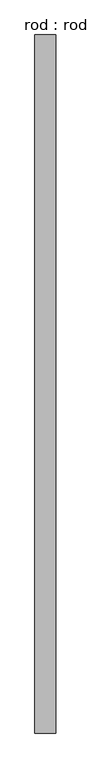
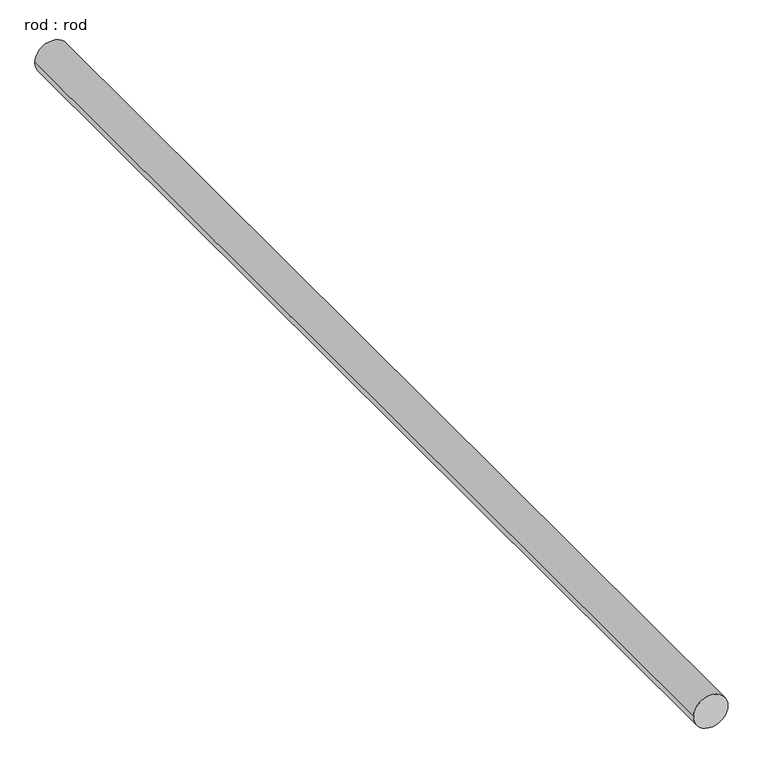
"""IFC4 building model written with IfcOpenShell, lengths in millimetres: proxy geometry, rod : rod."""

import ifcopenshell
import ifcopenshell.guid

model = None  # the IFC model being written
_history = None  # IfcOwnerHistory: only IFC2X3 demands one
_inside = {}  # id of a spatial element -> (the spatial element, [elements in it])
_under = {}  # id of a project, library or spatial element -> (it, [spatial elements below it])
_declared = {}  # id of a project -> (the project, [libraries it declares])
_typed = {}  # id of a type object -> (the type object, [elements of that type])
_made_of = {}  # id of a material, layer set ... -> (it, [elements and type objects made of it])


def new_model(schema):
    """Start an empty IFC model of exactly this schema.

    Asked for "IFC4X3", IfcOpenShell would pick the latest addendum, in which some entities
    have other attributes; the version numbers below select the first issue.
    IFC2X3 requires an IfcOwnerHistory on every rooted entity: one is made here for all.
    """
    global model, _history
    if schema == "IFC4X3":
        model = ifcopenshell.file(schema_version=(4, 3, 0, 0))
    else:
        model = ifcopenshell.file(schema=schema)
    _inside.clear()
    _under.clear()
    _declared.clear()
    _typed.clear()
    _made_of.clear()
    _history = None
    if model.schema == "IFC2X3":
        org = make("IfcOrganization", Name="unknown")
        user = make(
            "IfcPersonAndOrganization",
            ThePerson=make("IfcPerson", FamilyName="unknown"),
            TheOrganization=org,
        )
        app = make(
            "IfcApplication",
            ApplicationDeveloper=org,
            Version="unknown",
            ApplicationFullName="unknown",
            ApplicationIdentifier="unknown",
        )
        _history = make(
            "IfcOwnerHistory",
            OwningUser=user,
            OwningApplication=app,
            ChangeAction="ADDED",
            CreationDate=0,
        )
    return model


def make(cls, **values):
    """One entity of the class cls with the attributes given. An attribute that is None is left unset."""
    return model.create_entity(
        cls, **{name: value for name, value in values.items() if value is not None}
    )


def rooted(cls, **values):
    """An entity with a GlobalId (a new one), such as an element, a storey or a relation."""
    return make(cls, GlobalId=ifcopenshell.guid.new(), OwnerHistory=_history, **values)


def si_unit(unit_type, name, prefix=None):
    """IfcSIUnit, for example si_unit("LENGTHUNIT", "METRE", prefix="MILLI")."""
    return make("IfcSIUnit", UnitType=unit_type, Prefix=prefix, Name=name)


def assignment(units):
    """IfcUnitAssignment: the units of a project."""
    return None if units is None else make("IfcUnitAssignment", Units=units)


def point(xyz):
    """IfcCartesianPoint."""
    return None if xyz is None else make("IfcCartesianPoint", Coordinates=xyz)


def direction(xyz):
    """IfcDirection."""
    return None if xyz is None else make("IfcDirection", DirectionRatios=xyz)


def frame(location, z_axis=None, x_axis=None):
    """IfcAxis2Placement3D, a coordinate frame: its origin and axes. An axis left out is left unset."""
    return make(
        "IfcAxis2Placement3D",
        Location=point(location),
        Axis=direction(z_axis),
        RefDirection=direction(x_axis),
    )


def frame_2d(location, x_axis=None):
    """IfcAxis2Placement2D, a coordinate frame in the plane: its origin and x axis."""
    return make(
        "IfcAxis2Placement2D", Location=point(location), RefDirection=direction(x_axis)
    )


def origin():
    """The frame at (0, 0, 0) with its axes left unset."""
    return frame((0.0, 0.0, 0.0))


def place(relative_to, where):
    """IfcLocalPlacement: puts the frame where relative to a parent placement (None: the world)."""
    return make(
        "IfcLocalPlacement", PlacementRelTo=relative_to, RelativePlacement=where
    )


def context(
    kind, dimensions, precision=None, world=None, true_north=None, identifier=None
):
    """IfcGeometricRepresentationContext, for example the 3D "Model" context."""
    return make(
        "IfcGeometricRepresentationContext",
        ContextIdentifier=identifier,
        ContextType=kind,
        CoordinateSpaceDimension=dimensions,
        Precision=precision,
        WorldCoordinateSystem=world,
        TrueNorth=true_north,
    )


def project(units=None, contexts=None):
    """IfcProject with its units and contexts."""
    return rooted(
        "IfcProject",
        Name="project",
        RepresentationContexts=contexts,
        UnitsInContext=assignment(units),
    )


def spatial(cls, under=None, at=None, **own):
    """A site, building, storey or space (cls), placed at a placement, below another one or the project."""
    s = rooted(cls, ObjectPlacement=at, **own)
    if under is not None:
        _under.setdefault(under.id(), (under, []))[1].append(s)
    return s


def circle_curve(where, radius):
    """IfcCircle in the frame where."""
    return make("IfcCircle", Position=where, Radius=radius)


def trimmed(basis, trim1, trim2, sense, master):
    """IfcTrimmedCurve: the piece of a basis curve between two trims."""
    return make(
        "IfcTrimmedCurve",
        BasisCurve=basis,
        Trim1=trim1,
        Trim2=trim2,
        SenseAgreement=sense,
        MasterRepresentation=master,
    )


def segment(curve, same_sense, transition):
    """IfcCompositeCurveSegment."""
    return make(
        "IfcCompositeCurveSegment",
        Transition=transition,
        SameSense=same_sense,
        ParentCurve=curve,
    )


def composite_curve(segments, self_intersect=None):
    """IfcCompositeCurve: segments joined end to end."""
    return make("IfcCompositeCurve", Segments=segments, SelfIntersect=self_intersect)


def outline(outer, holes=None, kind="AREA"):
    """IfcArbitraryClosedProfileDef: a profile drawn as a closed curve; with holes, ...WithVoids."""
    if holes is None:
        return make("IfcArbitraryClosedProfileDef", ProfileType=kind, OuterCurve=outer)
    return make(
        "IfcArbitraryProfileDefWithVoids",
        ProfileType=kind,
        OuterCurve=outer,
        InnerCurves=holes,
    )


def extrude(swept, where, along, depth):
    """IfcExtrudedAreaSolid: the profile swept, set in the frame where, extruded along a direction by depth."""
    return make(
        "IfcExtrudedAreaSolid",
        SweptArea=swept,
        Position=where,
        ExtrudedDirection=direction(along),
        Depth=depth,
    )


def shape(context_of_items, identifier, shape_type, items):
    """IfcShapeRepresentation: the items that make up one representation, for example the "Body"."""
    return make(
        "IfcShapeRepresentation",
        ContextOfItems=context_of_items,
        RepresentationIdentifier=identifier,
        RepresentationType=shape_type,
        Items=items,
    )


def source(mapping_origin, context_of_items, identifier, shape_type, items):
    """IfcRepresentationMap: a shape defined once, which mapped items show again and again."""
    return make(
        "IfcRepresentationMap",
        MappingOrigin=mapping_origin,
        MappedRepresentation=shape(context_of_items, identifier, shape_type, items),
    )


def transform(
    local_origin,
    x_axis=None,
    y_axis=None,
    z_axis=None,
    scale=None,
    scale2=None,
    scale3=None,
    uniform=True,
):
    """IfcCartesianTransformationOperator3D, or its non-uniform kind. x_axis, y_axis, z_axis: its Axis1, 2, 3."""
    if uniform:
        return make(
            "IfcCartesianTransformationOperator3D",
            Axis1=direction(x_axis),
            Axis2=direction(y_axis),
            LocalOrigin=point(local_origin),
            Scale=scale,
            Axis3=direction(z_axis),
        )
    return make(
        "IfcCartesianTransformationOperator3DnonUniform",
        Axis1=direction(x_axis),
        Axis2=direction(y_axis),
        LocalOrigin=point(local_origin),
        Scale=scale,
        Axis3=direction(z_axis),
        Scale2=scale2,
        Scale3=scale3,
    )


def mapped(mapping_source, mapping_target):
    """IfcMappedItem: shows the shape of a source again, moved by a transform."""
    return make(
        "IfcMappedItem", MappingSource=mapping_source, MappingTarget=mapping_target
    )


def made_of(thing, what):
    """Note that an element or type object is made of a material, layer set ...; save() writes the relation."""
    if what is not None:
        _made_of.setdefault(what.id(), (what, []))[1].append(thing)
    return thing


def element(
    cls,
    number,
    at=None,
    inside=None,
    cuts=None,
    type_object=None,
    material=None,
    context=None,
    identifier="Body",
    shape_type=None,
    held_by="IfcProductDefinitionShape",
    body=None,
    shapes=None,
    **own,
):
    """One element of the class cls, such as IfcWall. Its Tag is "e" and its number.

    at: its placement. inside: the storey or other place that contains it. cuts: it is an
    opening in that element (IfcRelVoidsElement). A single representation is given by context,
    identifier, shape_type and body (its items); several are given by shapes. held_by: the class
    of the entity that holds the representations. save() writes the other relations.
    """
    e = rooted(cls, Tag="e%d" % number, ObjectPlacement=at, **own)
    if body is not None:
        shapes = [shape(context, identifier, shape_type, body)]
    if shapes is not None:
        e.Representation = make(held_by, Representations=shapes)
    if inside is not None:
        _inside.setdefault(inside.id(), (inside, []))[1].append(e)
    if cuts is not None:
        rooted(
            "IfcRelVoidsElement", RelatingBuildingElement=cuts, RelatedOpeningElement=e
        )
    if type_object is not None:
        _typed.setdefault(type_object.id(), (type_object, []))[1].append(e)
    return made_of(e, material)


def aggregate(whole, parts):
    """IfcRelAggregates: a whole, such as a stair, and the parts it consists of."""
    return rooted("IfcRelAggregates", RelatingObject=whole, RelatedObjects=parts)


def save(model, path):
    """Write the relations noted so far, then the file.

    IfcRelAggregates (storeys below a building ...), IfcRelContainedInSpatialStructure (elements
    in a storey), IfcRelDefinesByType, IfcRelAssociatesMaterial and IfcRelDeclares: one each for
    every whole, place, type object, material and project.
    """
    for whole, parts in _under.values():
        aggregate(whole, parts)
    for where, things in _inside.values():
        rooted(
            "IfcRelContainedInSpatialStructure",
            RelatedElements=things,
            RelatingStructure=where,
        )
    for kind, things in _typed.values():
        rooted("IfcRelDefinesByType", RelatedObjects=things, RelatingType=kind)
    for what, things in _made_of.values():
        rooted("IfcRelAssociatesMaterial", RelatedObjects=things, RelatingMaterial=what)
    for by, libraries in _declared.values():
        rooted("IfcRelDeclares", RelatingContext=by, RelatedDefinitions=libraries)
    model.write(path)


def rod_rod_481c27a9(model_context):
    return source(origin(), model_context, "Body", "SweptSolid", [
        extrude(outline(composite_curve([segment(trimmed(circle_curve(frame_2d((0.0108462, 0.0)), 200.0), [point((0.0108462, 200.0))], [point((0.0108462, -200.0))], False, "CARTESIAN"), True, "CONTINUOUS"), segment(trimmed(circle_curve(frame_2d((0.0108462, 0.0)), 200.0), [point((0.0108462, -200.0))], [point((0.0108462, 200.0))], False, "CARTESIAN"), True, "CONTINUOUS")], self_intersect=False)), frame((0.0, -2557.2713847, 0.0), z_axis=(0.0, 1.0, 0.0), x_axis=(0.0, 0.0, 1.0)), (0.0, 0.0, 1.0), 13300.0),
    ])


if __name__ == "__main__":
    model = new_model("IFC4")
    model_context = context("Model", 3, world=origin())
    ifc_project = project(units=[si_unit("LENGTHUNIT", "METRE", prefix="MILLI")], contexts=[model_context])
    site = spatial("IfcSite", under=ifc_project)
    building = spatial("IfcBuilding", under=site)
    placement = place(None, origin())
    rod_rod_shape = rod_rod_481c27a9(model_context)
    element("IfcBuildingElementProxy", 1, Name="rod : rod", ObjectType="rod : rod", at=placement, inside=building, context=model_context, shape_type="MappedRepresentation", body=[
        mapped(rod_rod_shape, transform((0.0, 0.0, 0.0), x_axis=(1.0, 0.0, 0.0), y_axis=(0.0, 1.0, 0.0), z_axis=(0.0, 0.0, 1.0))),
    ])
    save(model, "model.ifc")

# Revit data of these elements
# Type "rod : rod"
#   Default Elevation = 0
